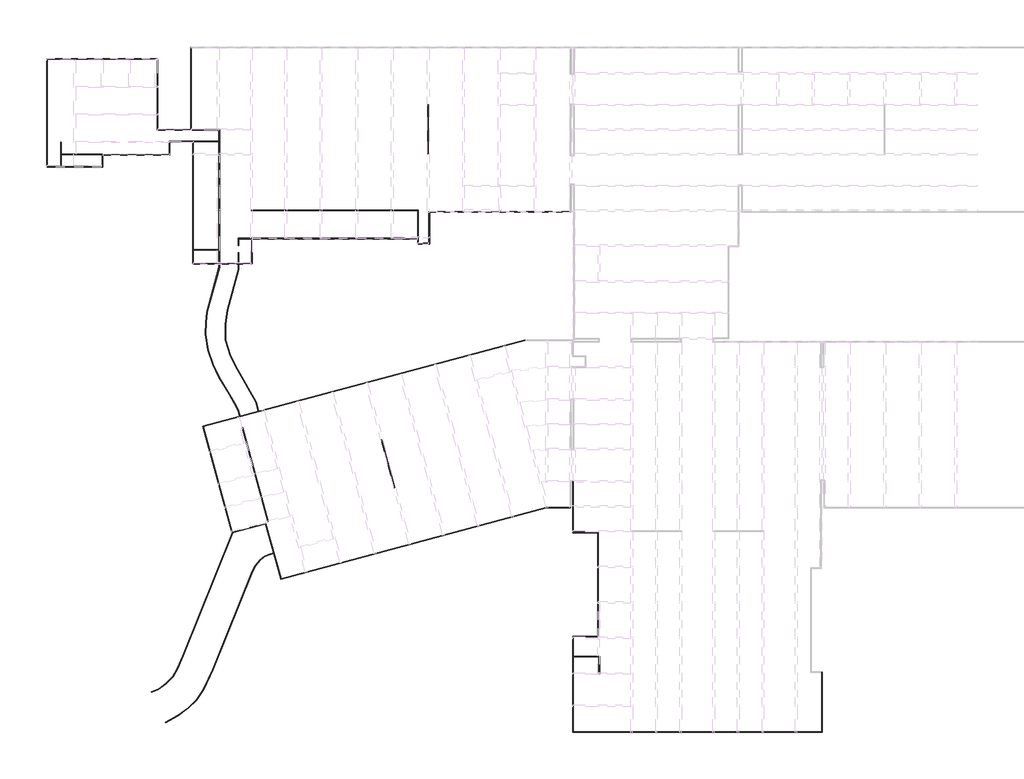
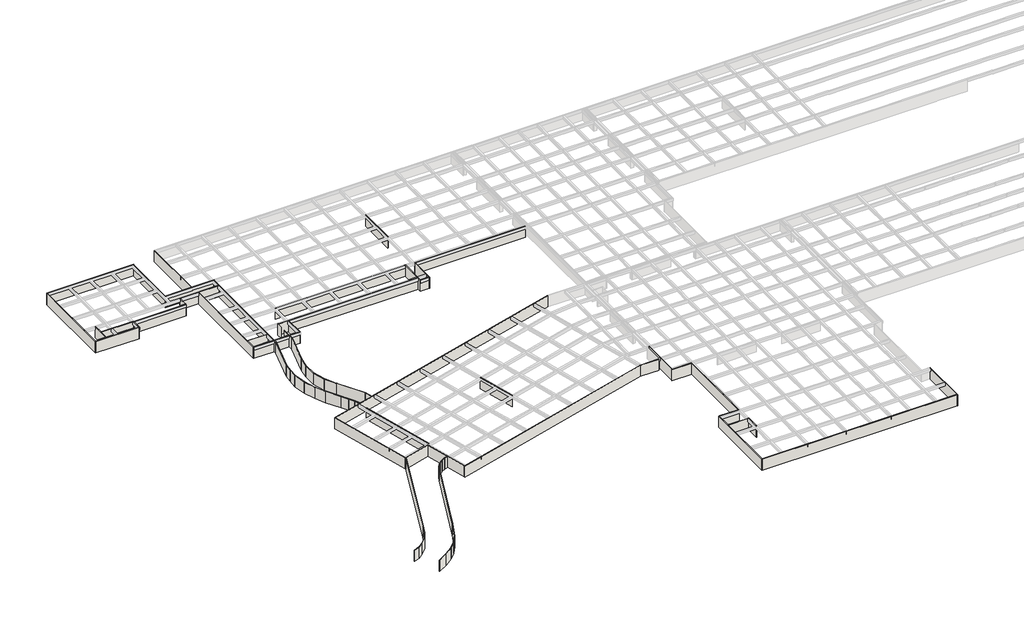
# One storey, part 1 of 14: 79 walls.
"""IFC4 building model written with IfcOpenShell, lengths in millimetres."""

from ifc_helpers import new_model, si_unit, origin, origin_with_axes, place, context, project, spatial, polyline, outline, extrude, faceted_brep, element, save

model = new_model("IFC4")

# Units and contexts
model_context = context("Model", 3, world=origin())
ifc_project = project(units=[si_unit("LENGTHUNIT", "METRE", prefix="MILLI")], contexts=[model_context])

# Site, building, storey
site = spatial("IfcSite", under=ifc_project)
building = spatial("IfcBuilding", under=site)
storey = spatial("IfcBuildingStorey", under=building, Name="户型图", Elevation=0.0)

# Walls
placement = place(None, origin())
element("IfcWall", 1, ObjectType="所有墙体", at=placement, inside=storey, context=model_context, shape_type="Brep", body=[
    faceted_brep([(-102060.8485237, -119994.1750557, 0.0), (-101940.8485237, -119994.1750557, 0.0), (-77810.8485237, -119994.1750557, 0.0), (-77690.8485237, -119994.1750557, 0.0), (-77690.8485237, -119994.1750557, 3300.0), (-77810.8485237, -119994.1750557, 3300.0), (-101940.8485237, -119994.1750557, 3300.0), (-102060.8485237, -119994.1750557, 3300.0), (-102060.8485237, -119874.1750557, 0.0), (-102060.8485237, -119874.1750557, 3300.0), (-77690.8485237, -119874.1750557, 3300.0), (-77690.8485237, -119874.1750557, 0.0)], [[[0, 1, 2, 3, 4, 5, 6, 7]], [[8, 9, 10, 11]], [[3, 2, 1, 0, 8, 11]], [[7, 6, 5, 4, 10, 9]], [[4, 3, 11, 10]], [[0, 7, 9, 8]]]),
])
element("IfcWall", 2, ObjectType="所有墙体", at=placement, inside=storey, context=model_context, shape_type="Brep", body=[
    faceted_brep([(-64072.7050956, -135348.950757, 0.0), (-70312.7050956, -135348.950757, 0.0), (-70432.7050956, -135348.950757, 0.0), (-77690.8485237, -135348.950757, 0.0), (-77810.8485237, -135348.950757, 0.0), (-77810.8485237, -135348.950757, 3300.0), (-77690.8485237, -135348.950757, 3300.0), (-70432.7050956, -135348.950757, 3300.0), (-70312.7050956, -135348.950757, 3300.0), (-64072.7050956, -135348.950757, 3300.0), (-64072.7050956, -135468.950757, 0.0), (-64072.7050956, -135468.950757, 3300.0), (-64162.6267154, -135468.950757, 3300.0), (-64282.6267154, -135468.950757, 3300.0), (-77810.8485237, -135468.950757, 3300.0), (-77810.8485237, -135468.950757, 0.0), (-64282.6267154, -135468.950757, 0.0), (-64162.6267154, -135468.950757, 0.0)], [[[0, 1, 2, 3, 4, 5, 6, 7, 8, 9]], [[10, 11, 12, 13, 14, 15, 16, 17]], [[4, 3, 2, 1, 0, 10, 17, 16, 15]], [[9, 8, 7, 6, 5, 14, 13, 12, 11]], [[0, 9, 11, 10]], [[5, 4, 15, 14]]]),
])
element("IfcWall", 3, ObjectType="所有墙体", at=placement, inside=storey, context=model_context, shape_type="SweptSolid", body=[
    extrude(outline(polyline([(-77690.8485237, -119994.1750557), (-77690.8485237, -135348.950757), (-77810.8485237, -135348.950757), (-77810.8485237, -119994.1750557), (-77690.8485237, -119994.1750557)])), origin_with_axes(), (0.0, 0.0, 1.0), 3300.0),
])
element("IfcWall", 4, ObjectType="所有墙体", at=placement, inside=storey, context=model_context, shape_type="Brep", body=[
    faceted_brep([(-64322.6267154, -137873.950757, 0.0), (-75185.8485237, -137873.950757, 0.0), (-75185.8485237, -137873.950757, 3300.0), (-64322.6267154, -137873.950757, 3300.0), (-64322.6267154, -137993.950757, 0.0), (-64322.6267154, -137993.950757, 3300.0), (-69912.7050956, -137993.950757, 3300.0), (-70032.7050956, -137993.950757, 3300.0), (-75065.8485237, -137993.950757, 3300.0), (-75185.8485237, -137993.950757, 3300.0), (-75185.8485237, -137993.950757, 0.0), (-75065.8485237, -137993.950757, 0.0), (-70032.7050956, -137993.950757, 0.0), (-69912.7050956, -137993.950757, 0.0)], [[[0, 1, 2, 3]], [[4, 5, 6, 7, 8, 9, 10, 11, 12, 13]], [[1, 0, 4, 13, 12, 11, 10]], [[3, 2, 9, 8, 7, 6, 5]], [[0, 3, 5, 4]], [[2, 1, 10, 9]]]),
])
element("IfcWall", 5, ObjectType="所有墙体", at=placement, inside=storey, context=model_context, shape_type="Brep", body=[
    faceted_brep([(-75185.8485237, -137993.950757, 0.0), (-75185.8485237, -140873.950757, 0.0), (-75185.8485237, -140993.950757, 0.0), (-75185.8485237, -140993.950757, 3300.0), (-75185.8485237, -140873.950757, 3300.0), (-75185.8485237, -137993.950757, 3300.0), (-75065.8485237, -137993.950757, 0.0), (-75065.8485237, -137993.950757, 3300.0), (-75065.8485237, -140993.950757, 3300.0), (-75065.8485237, -140993.950757, 0.0)], [[[0, 1, 2, 3, 4, 5]], [[6, 7, 8, 9]], [[2, 1, 0, 6, 9]], [[5, 4, 3, 8, 7]], [[0, 5, 7, 6]], [[3, 2, 9, 8]]]),
])
element("IfcWall", 6, ObjectType="所有墙体", at=placement, inside=storey, context=model_context, shape_type="Brep", body=[
    faceted_brep([(-75185.8485237, -140873.950757, 0.0), (-89885.8485237, -140873.950757, 0.0), (-89885.8485237, -140873.950757, 3300.0), (-75185.8485237, -140873.950757, 3300.0), (-75185.8485237, -140993.950757, 0.0), (-75185.8485237, -140993.950757, 3300.0), (-89765.8485237, -140993.950757, 3300.0), (-89885.8485237, -140993.950757, 3300.0), (-89885.8485237, -140993.950757, 0.0), (-89765.8485237, -140993.950757, 0.0)], [[[0, 1, 2, 3]], [[4, 5, 6, 7, 8, 9]], [[1, 0, 4, 9, 8]], [[3, 2, 7, 6, 5]], [[0, 3, 5, 4]], [[2, 1, 8, 7]]]),
])
element("IfcWall", 7, ObjectType="所有墙体", at=placement, inside=storey, context=model_context, shape_type="Brep", body=[
    faceted_brep([(-89885.8485237, -140993.950757, 0.0), (-89885.8485237, -143523.950757, 0.0), (-89885.8485237, -143643.950757, 0.0), (-89885.8485237, -143643.950757, 3300.0), (-89885.8485237, -143523.950757, 3300.0), (-89885.8485237, -140993.950757, 3300.0), (-89765.8485237, -140993.950757, 0.0), (-89765.8485237, -140993.950757, 3300.0), (-89765.8485237, -143643.950757, 3300.0), (-89765.8485237, -143643.950757, 0.0)], [[[0, 1, 2, 3, 4, 5]], [[6, 7, 8, 9]], [[2, 1, 0, 6, 9]], [[5, 4, 3, 8, 7]], [[0, 5, 7, 6]], [[3, 2, 9, 8]]]),
])
element("IfcWall", 8, ObjectType="所有墙体", at=placement, inside=storey, context=model_context, shape_type="Brep", body=[
    faceted_brep([(-89885.8485237, -143523.950757, 0.0), (-101940.8485237, -143523.950757, 0.0), (-102060.8485237, -143523.950757, 0.0), (-102060.8485237, -143523.950757, 3300.0), (-101940.8485237, -143523.950757, 3300.0), (-89885.8485237, -143523.950757, 3300.0), (-89885.8485237, -143643.950757, 0.0), (-89885.8485237, -143643.950757, 3300.0), (-102060.8485237, -143643.950757, 3300.0), (-102060.8485237, -143643.950757, 0.0)], [[[0, 1, 2, 3, 4, 5]], [[6, 7, 8, 9]], [[2, 1, 0, 6, 9]], [[5, 4, 3, 8, 7]], [[0, 5, 7, 6]], [[3, 2, 9, 8]]]),
])
element("IfcWall", 9, ObjectType="所有墙体", at=placement, inside=storey, context=model_context, shape_type="SweptSolid", body=[
    extrude(outline(polyline([(-101940.8485237, -119994.1750557), (-101940.8485237, -143523.950757), (-102060.8485237, -143523.950757), (-102060.8485237, -119994.1750557), (-101940.8485237, -119994.1750557)])), origin_with_axes(), (0.0, 0.0, 1.0), 3300.0),
])
element("IfcWall", 10, ObjectType="所有墙体", at=placement, inside=storey, context=model_context, shape_type="Brep", body=[
    faceted_brep([(-70312.7050956, -135348.950757, 0.0), (-70312.7050956, -117418.950757, 0.0), (-70312.7050956, -117298.950757, 0.0), (-70312.7050956, -117298.950757, 3300.0), (-70312.7050956, -117418.950757, 3300.0), (-70312.7050956, -135348.950757, 3300.0), (-70432.7050956, -135348.950757, 0.0), (-70432.7050956, -135348.950757, 3300.0), (-70432.7050956, -117298.950757, 3300.0), (-70432.7050956, -117298.950757, 0.0)], [[[0, 1, 2, 3, 4, 5]], [[6, 7, 8, 9]], [[2, 1, 0, 6, 9]], [[5, 4, 3, 8, 7]], [[0, 5, 7, 6]], [[3, 2, 9, 8]]]),
])
element("IfcWall", 11, ObjectType="所有墙体", at=placement, inside=storey, context=model_context, shape_type="Brep", body=[
    faceted_brep([(67772.2743803, -254333.1116625, 0.0), (67772.2743803, -267413.1116625, 0.0), (67772.2743803, -267533.1116625, 0.0), (67772.2743803, -267533.1116625, 3300.0), (67772.2743803, -267413.1116625, 3300.0), (67772.2743803, -254333.1116625, 3300.0), (67892.2743803, -254333.1116625, 0.0), (67892.2743803, -254333.1116625, 3300.0), (67892.2743803, -267533.1116625, 3300.0), (67892.2743803, -267533.1116625, 0.0)], [[[0, 1, 2, 3, 4, 5]], [[6, 7, 8, 9]], [[2, 1, 0, 6, 9]], [[5, 4, 3, 8, 7]], [[0, 5, 7, 6]], [[3, 2, 9, 8]]]),
])
element("IfcWall", 12, ObjectType="所有墙体", at=placement, inside=storey, context=model_context, shape_type="Brep", body=[
    faceted_brep([(67772.2743803, -267413.1116625, 0.0), (13292.2743803, -267413.1116625, 0.0), (13172.2743803, -267413.1116625, 0.0), (13172.2743803, -267413.1116625, 3300.0), (13292.2743803, -267413.1116625, 3300.0), (67772.2743803, -267413.1116625, 3300.0), (67772.2743803, -267533.1116625, 0.0), (67772.2743803, -267533.1116625, 3300.0), (13172.2743803, -267533.1116625, 3300.0), (13172.2743803, -267533.1116625, 0.0)], [[[0, 1, 2, 3, 4, 5]], [[6, 7, 8, 9]], [[2, 1, 0, 6, 9]], [[5, 4, 3, 8, 7]], [[0, 5, 7, 6]], [[3, 2, 9, 8]]]),
])
element("IfcWall", 13, ObjectType="所有墙体", at=placement, inside=storey, context=model_context, shape_type="Brep", body=[
    faceted_brep([(13292.2743803, -267413.1116625, 0.0), (13292.2743803, -250918.9547016, 0.0), (13292.2743803, -250798.9547016, 0.0), (13292.2743803, -246533.1116625, 0.0), (13292.2743803, -246413.1116625, 0.0), (13292.2743803, -246413.1116625, 3300.0), (13292.2743803, -246533.1116625, 3300.0), (13292.2743803, -250798.9547016, 3300.0), (13292.2743803, -250918.9547016, 3300.0), (13292.2743803, -267413.1116625, 3300.0), (13172.2743803, -267413.1116625, 0.0), (13172.2743803, -267413.1116625, 3300.0), (13172.2743803, -246413.1116625, 3300.0), (13172.2743803, -246413.1116625, 0.0)], [[[0, 1, 2, 3, 4, 5, 6, 7, 8, 9]], [[10, 11, 12, 13]], [[4, 3, 2, 1, 0, 10, 13]], [[9, 8, 7, 6, 5, 12, 11]], [[0, 9, 11, 10]], [[5, 4, 13, 12]]]),
])
element("IfcWall", 14, ObjectType="所有墙体", at=placement, inside=storey, context=model_context, shape_type="Brep", body=[
    faceted_brep([(13292.2743803, -246533.1116625, 0.0), (18792.2743803, -246533.1116625, 0.0), (18792.2743803, -246533.1116625, 3300.0), (13292.2743803, -246533.1116625, 3300.0), (13292.2743803, -246413.1116625, 0.0), (13292.2743803, -246413.1116625, 3300.0), (18672.2743803, -246413.1116625, 3300.0), (18792.2743803, -246413.1116625, 3300.0), (18792.2743803, -246413.1116625, 0.0), (18672.2743803, -246413.1116625, 0.0)], [[[0, 1, 2, 3]], [[4, 5, 6, 7, 8, 9]], [[1, 0, 4, 9, 8]], [[3, 2, 7, 6, 5]], [[0, 3, 5, 4]], [[2, 1, 8, 7]]]),
])
element("IfcWall", 15, ObjectType="所有墙体", at=placement, inside=storey, context=model_context, shape_type="Brep", body=[
    faceted_brep([(18792.2743803, -246413.1116625, 0.0), (18792.2743803, -223613.1116625, 0.0), (18792.2743803, -223613.1116625, 3300.0), (18792.2743803, -246413.1116625, 3300.0), (18672.2743803, -246413.1116625, 0.0), (18672.2743803, -246413.1116625, 3300.0), (18672.2743803, -223733.1116625, 3300.0), (18672.2743803, -223613.1116625, 3300.0), (18672.2743803, -223613.1116625, 0.0), (18672.2743803, -223733.1116625, 0.0)], [[[0, 1, 2, 3]], [[4, 5, 6, 7, 8, 9]], [[1, 0, 4, 9, 8]], [[3, 2, 7, 6, 5]], [[0, 3, 5, 4]], [[2, 1, 8, 7]]]),
])
element("IfcWall", 16, ObjectType="所有墙体", at=placement, inside=storey, context=model_context, shape_type="Brep", body=[
    faceted_brep([(18672.2743803, -223613.1116625, 0.0), (13292.2743803, -223613.1116625, 0.0), (13172.2743803, -223613.1116625, 0.0), (13172.2743803, -223613.1116625, 3300.0), (13292.2743803, -223613.1116625, 3300.0), (18672.2743803, -223613.1116625, 3300.0), (18672.2743803, -223733.1116625, 0.0), (18672.2743803, -223733.1116625, 3300.0), (13172.2743803, -223733.1116625, 3300.0), (13172.2743803, -223733.1116625, 0.0)], [[[0, 1, 2, 3, 4, 5]], [[6, 7, 8, 9]], [[2, 1, 0, 6, 9]], [[5, 4, 3, 8, 7]], [[0, 5, 7, 6]], [[3, 2, 9, 8]]]),
])
element("IfcWall", 17, ObjectType="所有墙体", at=placement, inside=storey, context=model_context, shape_type="Brep", body=[
    faceted_brep([(13292.2743803, -223613.1116625, 0.0), (13292.2743803, -212513.1116625, 0.0), (13292.2743803, -212513.1116625, 3300.0), (13292.2743803, -223613.1116625, 3300.0), (13172.2743803, -223613.1116625, 0.0), (13172.2743803, -223613.1116625, 3300.0), (13172.2743803, -212633.1116625, 3300.0), (13172.2743803, -212513.1116625, 3300.0), (13172.2743803, -212513.1116625, 0.0), (13172.2743803, -212633.1116625, 0.0)], [[[0, 1, 2, 3]], [[4, 5, 6, 7, 8, 9]], [[1, 0, 4, 9, 8]], [[3, 2, 7, 6, 5]], [[0, 3, 5, 4]], [[2, 1, 8, 7]]]),
])
element("IfcWall", 18, ObjectType="所有墙体", at=placement, inside=storey, context=model_context, shape_type="SweptSolid", body=[
    extrude(outline(polyline([(7424.3695711, -218205.2956278), (12672.2743803, -218205.2956278), (12672.2743803, -218325.2956278), (7440.1791895, -218325.2956278), (7424.3695711, -218205.2956278)])), origin_with_axes(), (0.0, 0.0, 1.0), 3300.0),
])
element("IfcWall", 19, ObjectType="所有墙体", at=placement, inside=storey, context=model_context, shape_type="Brep", body=[
    faceted_brep([(7424.3695711, -218205.2956278, 0.0), (-50671.4297883, -233783.5648272, 0.0), (-50787.3364124, -233814.6449502, 0.0), (-50787.3364124, -233814.6449502, 3300.0), (-50671.4297883, -233783.5648272, 3300.0), (7424.3695711, -218205.2956278, 3300.0), (7440.1791895, -218325.2956278, 0.0), (7440.1791895, -218325.2956278, 3300.0), (-50755.7106249, -233930.403877, 3300.0), (-50755.7106249, -233930.403877, 0.0)], [[[0, 1, 2, 3, 4, 5]], [[6, 7, 8, 9]], [[2, 1, 0, 6, 9]], [[5, 4, 3, 8, 7]], [[0, 5, 7, 6]], [[3, 2, 9, 8]]]),
])
element("IfcWall", 20, ObjectType="所有墙体", at=placement, inside=storey, context=model_context, shape_type="Brep", body=[
    faceted_brep([(-50671.4297883, -233783.5648272, 0.0), (-53985.8264316, -221651.9776687, 0.0), (-53985.8264316, -221651.9776687, 3300.0), (-50671.4297883, -233783.5648272, 3300.0), (-50787.3364124, -233814.6449502, 0.0), (-50787.3364124, -233814.6449502, 3300.0), (-52290.212691, -228313.7117417, 3300.0), (-52321.8387283, -228197.9519009, 3300.0), (-54070.1131044, -221798.7953563, 3300.0), (-54101.7389202, -221683.0363264, 3300.0), (-54101.7389202, -221683.0363264, 0.0), (-54070.1131044, -221798.7953563, 0.0), (-52321.8387283, -228197.9519009, 0.0), (-52290.212691, -228313.7117417, 0.0)], [[[0, 1, 2, 3]], [[4, 5, 6, 7, 8, 9, 10, 11, 12, 13]], [[1, 0, 4, 13, 12, 11, 10]], [[3, 2, 9, 8, 7, 6, 5]], [[0, 3, 5, 4]], [[2, 1, 10, 9]]]),
])
element("IfcWall", 21, ObjectType="所有墙体", at=placement, inside=storey, context=model_context, shape_type="Brep", body=[
    faceted_brep([(-54101.7389202, -221683.0363264, 0.0), (-61389.3646897, -223635.7497661, 0.0), (-61505.2771782, -223666.8084238, 0.0), (-61505.2771782, -223666.8084238, 3300.0), (-61389.3646897, -223635.7497661, 3300.0), (-54101.7389202, -221683.0363264, 3300.0), (-54070.1131044, -221798.7953563, 0.0), (-54070.1131044, -221798.7953563, 3300.0), (-61473.6513625, -223782.5674537, 3300.0), (-61473.6513625, -223782.5674537, 0.0)], [[[0, 1, 2, 3, 4, 5]], [[6, 7, 8, 9]], [[2, 1, 0, 6, 9]], [[5, 4, 3, 8, 7]], [[0, 5, 7, 6]], [[3, 2, 9, 8]]]),
])
element("IfcWall", 22, ObjectType="所有墙体", at=placement, inside=storey, context=model_context, shape_type="Brep", body=[
    faceted_brep([(-61389.3646897, -223635.7497661, 0.0), (-67709.1807348, -200503.5156291, 0.0), (-67740.8065505, -200387.7565992, 0.0), (-67740.8065505, -200387.7565992, 3300.0), (-67709.1807348, -200503.5156291, 3300.0), (-61389.3646897, -223635.7497661, 3300.0), (-61505.2771782, -223666.8084238, 0.0), (-61505.2771782, -223666.8084238, 3300.0), (-67856.719039, -200418.8152569, 3300.0), (-67856.719039, -200418.8152569, 0.0)], [[[0, 1, 2, 3, 4, 5]], [[6, 7, 8, 9]], [[2, 1, 0, 6, 9]], [[5, 4, 3, 8, 7]], [[0, 5, 7, 6]], [[3, 2, 9, 8]]]),
])
element("IfcWall", 23, ObjectType="所有墙体", at=placement, inside=storey, context=model_context, shape_type="Brep", body=[
    faceted_brep([(-67709.1807348, -200503.5156291, 0.0), (2737.534582, -181627.3751505, 0.0), (2737.534582, -181627.3751505, 3300.0), (-67709.1807348, -200503.5156291, 3300.0), (-67740.8065505, -200387.7565992, 0.0), (-67740.8065505, -200387.7565992, 3300.0), (-59754.9827385, -198247.9615579, 3300.0), (-59639.0716393, -198216.9032725, 3300.0), (-55640.8160452, -197145.5739149, 3300.0), (-55524.904946, -197114.5156295, 3300.0), (2721.7362823, -181507.3751505, 3300.0), (2721.7362823, -181507.3751505, 0.0), (-55524.904946, -197114.5156295, 0.0), (-55640.8160452, -197145.5739149, 0.0), (-59639.0716393, -198216.9032725, 0.0), (-59754.9827385, -198247.9615579, 0.0)], [[[0, 1, 2, 3]], [[4, 5, 6, 7, 8, 9, 10, 11, 12, 13, 14, 15]], [[1, 0, 4, 15, 14, 13, 12, 11]], [[3, 2, 10, 9, 8, 7, 6, 5]], [[0, 3, 5, 4]], [[2, 1, 11, 10]]]),
])
element("IfcWall", 24, ObjectType="所有墙体", at=placement, inside=storey, context=model_context, shape_type="Brep", body=[
    faceted_brep([(12717.2949044, -153307.3751505, 0.0), (-18282.7050956, -153307.3751505, 0.0), (-18282.7050956, -153307.3751505, 3300.0), (12717.2949044, -153307.3751505, 3300.0), (12717.2949044, -153427.3751505, 0.0), (12717.2949044, -153427.3751505, 3300.0), (-18162.7050956, -153427.3751505, 3300.0), (-18282.7050956, -153427.3751505, 3300.0), (-18282.7050956, -153427.3751505, 0.0), (-18162.7050956, -153427.3751505, 0.0)], [[[0, 1, 2, 3]], [[4, 5, 6, 7, 8, 9]], [[1, 0, 4, 9, 8]], [[3, 2, 7, 6, 5]], [[0, 3, 5, 4]], [[2, 1, 8, 7]]]),
])
element("IfcWall", 25, ObjectType="所有墙体", at=placement, inside=storey, context=model_context, shape_type="Brep", body=[
    faceted_brep([(-18282.7050956, -153427.3751505, 0.0), (-18282.7050956, -160307.3751505, 0.0), (-18282.7050956, -160427.3751505, 0.0), (-18282.7050956, -160427.3751505, 3300.0), (-18282.7050956, -160307.3751505, 3300.0), (-18282.7050956, -153427.3751505, 3300.0), (-18162.7050956, -153427.3751505, 0.0), (-18162.7050956, -153427.3751505, 3300.0), (-18162.7050956, -160427.3751505, 3300.0), (-18162.7050956, -160427.3751505, 0.0)], [[[0, 1, 2, 3, 4, 5]], [[6, 7, 8, 9]], [[2, 1, 0, 6, 9]], [[5, 4, 3, 8, 7]], [[0, 5, 7, 6]], [[3, 2, 9, 8]]]),
])
element("IfcWall", 26, ObjectType="所有墙体", at=placement, inside=storey, context=model_context, shape_type="Brep", body=[
    faceted_brep([(-18282.7050956, -160307.3751505, 0.0), (-20662.7050956, -160307.3751505, 0.0), (-20782.7050956, -160307.3751505, 0.0), (-20782.7050956, -160307.3751505, 3300.0), (-20662.7050956, -160307.3751505, 3300.0), (-18282.7050956, -160307.3751505, 3300.0), (-18282.7050956, -160427.3751505, 0.0), (-18282.7050956, -160427.3751505, 3300.0), (-20782.7050956, -160427.3751505, 3300.0), (-20782.7050956, -160427.3751505, 0.0)], [[[0, 1, 2, 3, 4, 5]], [[6, 7, 8, 9]], [[2, 1, 0, 6, 9]], [[5, 4, 3, 8, 7]], [[0, 5, 7, 6]], [[3, 2, 9, 8]]]),
])
element("IfcWall", 27, ObjectType="所有墙体", at=placement, inside=storey, context=model_context, shape_type="Brep", body=[
    faceted_brep([(-20662.7050956, -160307.3751505, 0.0), (-20662.7050956, -153048.950757, 0.0), (-20662.7050956, -153048.950757, 3300.0), (-20662.7050956, -160307.3751505, 3300.0), (-20782.7050956, -160307.3751505, 0.0), (-20782.7050956, -160307.3751505, 3300.0), (-20782.7050956, -159327.3751505, 3300.0), (-20782.7050956, -159207.3751505, 3300.0), (-20782.7050956, -153168.950757, 3300.0), (-20782.7050956, -153048.950757, 3300.0), (-20782.7050956, -153048.950757, 0.0), (-20782.7050956, -153168.950757, 0.0), (-20782.7050956, -159207.3751505, 0.0), (-20782.7050956, -159327.3751505, 0.0)], [[[0, 1, 2, 3]], [[4, 5, 6, 7, 8, 9, 10, 11, 12, 13]], [[1, 0, 4, 13, 12, 11, 10]], [[3, 2, 9, 8, 7, 6, 5]], [[0, 3, 5, 4]], [[2, 1, 10, 9]]]),
])
element("IfcWall", 28, ObjectType="所有墙体", at=placement, inside=storey, context=model_context, shape_type="Brep", body=[
    faceted_brep([(-20782.7050956, -159207.3751505, 0.0), (-59913.7017341, -159207.3751505, 0.0), (-59913.7017341, -159207.3751505, 3300.0), (-20782.7050956, -159207.3751505, 3300.0), (-20782.7050956, -159327.3751505, 0.0), (-20782.7050956, -159327.3751505, 3300.0), (-56962.7050956, -159327.3751505, 3300.0), (-57082.7050956, -159327.3751505, 3300.0), (-59913.7017341, -159327.3751505, 3300.0), (-59913.7017341, -159327.3751505, 0.0), (-57082.7050956, -159327.3751505, 0.0), (-56962.7050956, -159327.3751505, 0.0)], [[[0, 1, 2, 3]], [[4, 5, 6, 7, 8, 9, 10, 11]], [[1, 0, 4, 11, 10, 9]], [[3, 2, 8, 7, 6, 5]], [[0, 3, 5, 4]], [[2, 1, 9, 8]]]),
])
element("IfcWall", 29, ObjectType="所有墙体", at=placement, inside=storey, context=model_context, shape_type="Brep", body=[
    faceted_brep([(-57082.7050956, -159327.3751505, 0.0), (-57082.7050956, -164698.4277999, 0.0), (-57082.7050956, -164818.4277999, 0.0), (-57082.7050956, -164818.4277999, 3300.0), (-57082.7050956, -164698.4277999, 3300.0), (-57082.7050956, -159327.3751505, 3300.0), (-56962.7050956, -159327.3751505, 0.0), (-56962.7050956, -159327.3751505, 3300.0), (-56962.7050956, -164818.4277999, 3300.0), (-56962.7050956, -164818.4277999, 0.0)], [[[0, 1, 2, 3, 4, 5]], [[6, 7, 8, 9]], [[2, 1, 0, 6, 9]], [[5, 4, 3, 8, 7]], [[0, 5, 7, 6]], [[3, 2, 9, 8]]]),
])
element("IfcWall", 30, ObjectType="所有墙体", at=placement, inside=storey, context=model_context, shape_type="Brep", body=[
    faceted_brep([(-57082.7050956, -164698.4277999, 0.0), (-59950.6326698, -164698.4277999, 0.0), (-60070.6326698, -164698.4277999, 0.0), (-64162.6267154, -164698.4277999, 0.0), (-64282.6267154, -164698.4277999, 0.0), (-69912.7050956, -164698.4277999, 0.0), (-70032.7050956, -164698.4277999, 0.0), (-70032.7050956, -164698.4277999, 3300.0), (-69912.7050956, -164698.4277999, 3300.0), (-64282.6267154, -164698.4277999, 3300.0), (-64162.6267154, -164698.4277999, 3300.0), (-60070.6326698, -164698.4277999, 3300.0), (-59950.6326698, -164698.4277999, 3300.0), (-57082.7050956, -164698.4277999, 3300.0), (-57082.7050956, -164818.4277999, 0.0), (-57082.7050956, -164818.4277999, 3300.0), (-59950.6326698, -164818.4277999, 3300.0), (-60070.6326698, -164818.4277999, 3300.0), (-64162.6267154, -164818.4277999, 3300.0), (-64282.6267154, -164818.4277999, 3300.0), (-70032.7050956, -164818.4277999, 3300.0), (-70032.7050956, -164818.4277999, 0.0), (-64282.6267154, -164818.4277999, 0.0), (-64162.6267154, -164818.4277999, 0.0), (-60070.6326698, -164818.4277999, 0.0), (-59950.6326698, -164818.4277999, 0.0)], [[[0, 1, 2, 3, 4, 5, 6, 7, 8, 9, 10, 11, 12, 13]], [[14, 15, 16, 17, 18, 19, 20, 21, 22, 23, 24, 25]], [[6, 5, 4, 3, 2, 1, 0, 14, 25, 24, 23, 22, 21]], [[13, 12, 11, 10, 9, 8, 7, 20, 19, 18, 17, 16, 15]], [[0, 13, 15, 14]], [[7, 6, 21, 20]]]),
])
element("IfcWall", 31, ObjectType="所有墙体", at=placement, inside=storey, context=model_context, shape_type="Brep", body=[
    faceted_brep([(-69912.7050956, -164698.4277999, 0.0), (-69912.7050956, -161762.6341765, 0.0), (-69912.7050956, -161642.6341765, 0.0), (-69912.7050956, -137993.950757, 0.0), (-69912.7050956, -137993.950757, 3300.0), (-69912.7050956, -161642.6341765, 3300.0), (-69912.7050956, -161762.6341765, 3300.0), (-69912.7050956, -164698.4277999, 3300.0), (-70032.7050956, -164698.4277999, 0.0), (-70032.7050956, -164698.4277999, 3300.0), (-70032.7050956, -137993.950757, 3300.0), (-70032.7050956, -137993.950757, 0.0)], [[[0, 1, 2, 3, 4, 5, 6, 7]], [[8, 9, 10, 11]], [[3, 2, 1, 0, 8, 11]], [[7, 6, 5, 4, 10, 9]], [[0, 7, 9, 8]], [[4, 3, 11, 10]]]),
])
element("IfcWall", 32, ObjectType="所有墙体", at=placement, inside=storey, context=model_context, shape_type="SweptSolid", body=[
    extrude(outline(polyline([(-25928.9541564, -213876.8076269), (-28736.3690064, -203399.4100936), (-28620.4579201, -203368.3517603), (-25813.0430701, -213845.7492935), (-25928.9541564, -213876.8076269)])), origin_with_axes(), (0.0, 0.0, 1.0), 3300.0),
])
element("IfcWall", 33, ObjectType="所有墙体", at=placement, inside=storey, context=model_context, shape_type="SweptSolid", body=[
    extrude(outline(polyline([(-18534.1452268, -140660.1299915), (-18534.1452268, -129960.1299915), (-18414.1452268, -129960.1299915), (-18414.1452268, -140660.1299915), (-18534.1452268, -140660.1299915)])), origin_with_axes(), (0.0, 0.0, 1.0), 3300.0),
])
element("IfcWall", 34, ObjectType="所有墙体", at=placement, inside=storey, context=model_context, shape_type="SweptSolid", body=[
    extrude(outline(polyline([(-57172.7050956, -153048.950757), (-20782.7050956, -153048.950757), (-20782.7050956, -153168.950757), (-57172.7050956, -153168.950757), (-57172.7050956, -153048.950757)])), origin_with_axes(), (0.0, 0.0, 1.0), 3300.0),
])
element("IfcWall", 35, ObjectType="所有墙体", at=placement, inside=storey, context=model_context, shape_type="Brep", body=[
    faceted_brep([(-64282.6267154, -135468.950757, 0.0), (-64282.6267154, -161642.6341765, 0.0), (-64282.6267154, -161762.6341765, 0.0), (-64282.6267154, -164698.4277999, 0.0), (-64282.6267154, -164698.4277999, 3300.0), (-64282.6267154, -161762.6341765, 3300.0), (-64282.6267154, -161642.6341765, 3300.0), (-64282.6267154, -135468.950757, 3300.0), (-64162.6267154, -135468.950757, 0.0), (-64162.6267154, -135468.950757, 3300.0), (-64162.6267154, -164698.4277999, 3300.0), (-64162.6267154, -164698.4277999, 0.0)], [[[0, 1, 2, 3, 4, 5, 6, 7]], [[8, 9, 10, 11]], [[3, 2, 1, 0, 8, 11]], [[7, 6, 5, 4, 10, 9]], [[0, 7, 9, 8]], [[4, 3, 11, 10]]]),
])
element("IfcWall", 36, ObjectType="所有墙体", at=placement, inside=storey, context=model_context, shape_type="SweptSolid", body=[
    extrude(outline(polyline([(-69912.7050956, -161642.6341765), (-64282.6267154, -161642.6341765), (-64282.6267154, -161762.6341765), (-69912.7050956, -161762.6341765), (-69912.7050956, -161642.6341765)])), origin_with_axes(), (0.0, 0.0, 1.0), 3300.0),
])
element("IfcWall", 37, ObjectType="所有墙体", at=placement, inside=storey, context=model_context, shape_type="SweptSolid", body=[
    extrude(outline(polyline([(-64282.6267154, -165550.52865), (-64282.6267154, -164818.4277999), (-64162.6267154, -164818.4277999), (-64162.6267154, -165566.3269497), (-64282.6267154, -165550.52865)])), origin_with_axes(), (0.0, 0.0, 1.0), 3300.0),
])
element("IfcWall", 38, ObjectType="所有墙体", at=placement, inside=storey, context=model_context, shape_type="SweptSolid", body=[
    extrude(outline(polyline([(-66921.7586951, -175399.903286), (-64282.6267154, -165550.52865), (-64162.6267154, -165566.3269497), (-66803.4032558, -175421.83917), (-66921.7586951, -175399.903286)])), origin_with_axes(), (0.0, 0.0, 1.0), 3300.0),
])
element("IfcWall", 39, ObjectType="所有墙体", at=placement, inside=storey, context=model_context, shape_type="SweptSolid", body=[
    extrude(outline(polyline([(-67162.8319851, -177693.5624279), (-66921.7586951, -175399.903286), (-66803.4032558, -175421.83917), (-67043.1608968, -177702.9807468), (-67162.8319851, -177693.5624279)])), origin_with_axes(), (0.0, 0.0, 1.0), 3300.0),
])
element("IfcWall", 40, ObjectType="所有墙体", at=placement, inside=storey, context=model_context, shape_type="SweptSolid", body=[
    extrude(outline(polyline([(-67291.9097037, -180156.5120195), (-67162.8319851, -177693.5624279), (-67043.1608968, -177702.9807468), (-67171.4140719, -180150.197111), (-67291.9097037, -180156.5120195)])), origin_with_axes(), (0.0, 0.0, 1.0), 3300.0),
])
element("IfcWall", 41, ObjectType="所有墙体", at=placement, inside=storey, context=model_context, shape_type="SweptSolid", body=[
    extrude(outline(polyline([(-66726.9816527, -183723.3273571), (-67291.9097037, -180156.5120195), (-67171.4140719, -180150.197111), (-66610.0139746, -183694.7378257), (-66726.9816527, -183723.3273571)])), origin_with_axes(), (0.0, 0.0, 1.0), 3300.0),
])
element("IfcWall", 42, ObjectType="所有墙体", at=placement, inside=storey, context=model_context, shape_type="SweptSolid", body=[
    extrude(outline(polyline([(-65678.7698235, -186861.5323686), (-66726.9816527, -183723.3273571), (-66610.0139746, -183694.7378257), (-65567.2747284, -186816.5586607), (-65678.7698235, -186861.5323686)])), origin_with_axes(), (0.0, 0.0, 1.0), 3300.0),
])
element("IfcWall", 43, ObjectType="所有墙体", at=placement, inside=storey, context=model_context, shape_type="SweptSolid", body=[
    extrude(outline(polyline([(-64343.0654647, -189666.2881503), (-65678.7698235, -186861.5323686), (-65567.2747284, -186816.5586607), (-64237.2178441, -189609.4556902), (-64343.0654647, -189666.2881503)])), origin_with_axes(), (0.0, 0.0, 1.0), 3300.0),
])
element("IfcWall", 44, ObjectType="所有墙体", at=placement, inside=storey, context=model_context, shape_type="SweptSolid", body=[
    extrude(outline(polyline([(-62055.07232, -193474.1481968), (-64343.0654647, -189666.2881503), (-64237.2178441, -189609.4556902), (-61951.6728836, -193413.241274), (-62055.07232, -193474.1481968)])), origin_with_axes(), (0.0, 0.0, 1.0), 3300.0),
])
element("IfcWall", 45, ObjectType="所有墙体", at=placement, inside=storey, context=model_context, shape_type="SweptSolid", body=[
    extrude(outline(polyline([(-60955.4254517, -195378.7924431), (-62055.07232, -193474.1481967), (-61951.6728836, -193413.241274), (-60851.3197519, -195319.1088044), (-60955.4254517, -195378.7924431)])), origin_with_axes(), (0.0, 0.0, 1.0), 3300.0),
])
element("IfcWall", 46, ObjectType="所有墙体", at=placement, inside=storey, context=model_context, shape_type="SweptSolid", body=[
    extrude(outline(polyline([(-60139.9172399, -196811.3664409), (-60955.4254517, -195378.7924431), (-60851.3197519, -195319.1088044), (-60027.9988942, -196765.406997), (-60139.9172399, -196811.3664409)])), origin_with_axes(), (0.0, 0.0, 1.0), 3300.0),
])
element("IfcWall", 47, ObjectType="所有墙体", at=placement, inside=storey, context=model_context, shape_type="SweptSolid", body=[
    extrude(outline(polyline([(-59754.9827385, -198247.9615579), (-60139.9172399, -196811.3664409), (-60027.9988942, -196765.406997), (-59639.0716393, -198216.9032725), (-59754.9827385, -198247.9615579)])), origin_with_axes(), (0.0, 0.0, 1.0), 3300.0),
])
element("IfcWall", 48, ObjectType="所有墙体", at=placement, inside=storey, context=model_context, shape_type="SweptSolid", body=[
    extrude(outline(polyline([(-56080.8229941, -195039.8045814), (-55524.904946, -197114.5156295), (-55640.8160452, -197145.5739149), (-56192.6451801, -195086.1228739), (-56080.8229941, -195039.8045814)])), origin_with_axes(), (0.0, 0.0, 1.0), 3300.0),
])
element("IfcWall", 49, ObjectType="所有墙体", at=placement, inside=storey, context=model_context, shape_type="SweptSolid", body=[
    extrude(outline(polyline([(-60184.3356946, -187932.3120946), (-56080.8229941, -195039.8045814), (-56192.6451801, -195086.1228739), (-60289.1324796, -187990.7987386), (-60184.3356946, -187932.3120946)])), origin_with_axes(), (0.0, 0.0, 1.0), 3300.0),
])
element("IfcWall", 50, ObjectType="所有墙体", at=placement, inside=storey, context=model_context, shape_type="SweptSolid", body=[
    extrude(outline(polyline([(-61755.993167, -185017.256202), (-60184.3356946, -187932.3120946), (-60289.1324796, -187990.7987386), (-61867.4848403, -185063.3253989), (-61755.993167, -185017.256202)])), origin_with_axes(), (0.0, 0.0, 1.0), 3300.0),
])
element("IfcWall", 51, ObjectType="所有墙体", at=placement, inside=storey, context=model_context, shape_type="SweptSolid", body=[
    extrude(outline(polyline([(-62816.7147264, -181452.3559054), (-61755.993167, -185017.256202), (-61867.4848403, -185063.3253989), (-62936.7147264, -181469.830099), (-62816.7147264, -181452.3559054)])), origin_with_axes(), (0.0, 0.0, 1.0), 3300.0),
])
element("IfcWall", 52, ObjectType="所有墙体", at=placement, inside=storey, context=model_context, shape_type="SweptSolid", body=[
    extrude(outline(polyline([(-62816.7147264, -177965.8151046), (-62816.7147264, -181452.3559054), (-62936.7147264, -181469.830099), (-62936.7147264, -177956.3708998), (-62816.7147264, -177965.8151046)])), origin_with_axes(), (0.0, 0.0, 1.0), 3300.0),
])
element("IfcWall", 53, ObjectType="所有墙体", at=placement, inside=storey, context=model_context, shape_type="SweptSolid", body=[
    extrude(outline(polyline([(-62332.9984873, -174911.7509674), (-62816.7147264, -177965.8151046), (-62936.7147264, -177956.3708998), (-62450.5372822, -174886.7673253), (-62332.9984873, -174911.7509674)])), origin_with_axes(), (0.0, 0.0, 1.0), 3300.0),
])
element("IfcWall", 54, ObjectType="所有墙体", at=placement, inside=storey, context=model_context, shape_type="SweptSolid", body=[
    extrude(outline(polyline([(-59950.6326698, -166020.6406944), (-62332.9984873, -174911.7509674), (-62450.5372822, -174886.7673253), (-60070.6326698, -166004.8423946), (-59950.6326698, -166020.6406944)])), origin_with_axes(), (0.0, 0.0, 1.0), 3300.0),
])
element("IfcWall", 55, ObjectType="所有墙体", at=placement, inside=storey, context=model_context, shape_type="SweptSolid", body=[
    extrude(outline(polyline([(-59950.6326698, -164818.4277999), (-59950.6326698, -166020.6406944), (-60070.6326698, -166004.8423946), (-60070.6326698, -164818.4277999), (-59950.6326698, -164818.4277999)])), origin_with_axes(), (0.0, 0.0, 1.0), 3300.0),
])
element("IfcWall", 56, ObjectType="所有墙体", at=placement, inside=storey, context=model_context, shape_type="SweptSolid", body=[
    extrude(outline(polyline([(-59950.6326698, -162357.0185835), (-59950.6326698, -164698.4277999), (-60070.6326698, -164698.4277999), (-60070.6326698, -162357.0185835), (-59950.6326698, -162357.0185835)])), origin_with_axes(), (0.0, 0.0, 1.0), 3300.0),
])
element("IfcWall", 57, ObjectType="所有墙体", at=placement, inside=storey, context=model_context, shape_type="Brep", body=[
    faceted_brep([(-59913.7017341, -160829.181821, 0.0), (-59913.7017341, -159327.3751505, 0.0), (-59913.7017341, -159207.3751505, 0.0), (-59913.7017341, -159189.181821, 0.0), (-59913.7017341, -159189.181821, 3300.0), (-59913.7017341, -159207.3751505, 3300.0), (-59913.7017341, -159327.3751505, 3300.0), (-59913.7017341, -160829.181821, 3300.0), (-60033.7017341, -160829.181821, 0.0), (-60033.7017341, -160829.181821, 3300.0), (-60033.7017341, -159189.181821, 3300.0), (-60033.7017341, -159189.181821, 0.0)], [[[0, 1, 2, 3, 4, 5, 6, 7]], [[8, 9, 10, 11]], [[3, 2, 1, 0, 8, 11]], [[4, 3, 11, 10]], [[7, 6, 5, 4, 10, 9]], [[0, 7, 9, 8]]]),
])
element("IfcWall", 58, ObjectType="所有墙体", at=placement, inside=storey, context=model_context, shape_type="SweptSolid", body=[
    extrude(outline(polyline([(-59074.9933121, -200705.199268), (-53479.354271, -221257.0562089), (-53595.1393805, -221288.5809359), (-59190.7784216, -200736.723995), (-59074.9933121, -200705.199268)])), origin_with_axes(), (0.0, 0.0, 1.0), 3300.0),
])
element("IfcWall", 59, ObjectType="所有墙体", at=placement, inside=storey, context=model_context, shape_type="SweptSolid", body=[
    extrude(outline(polyline([(-53332.1758898, -228467.2995997), (-52321.8387283, -228197.9519009), (-52290.212691, -228313.7117417), (-53289.6794099, -228580.1614685), (-53332.1758898, -228467.2995997)])), origin_with_axes(), (0.0, 0.0, 1.0), 3300.0),
])
element("IfcWall", 60, ObjectType="所有墙体", at=placement, inside=storey, context=model_context, shape_type="SweptSolid", body=[
    extrude(outline(polyline([(-54384.4165476, -228988.2371362), (-53332.1758898, -228467.2995997), (-53289.6794099, -228580.1614685), (-54323.0312208, -229091.7476183), (-54384.4165476, -228988.2371362)])), origin_with_axes(), (0.0, 0.0, 1.0), 3300.0),
])
element("IfcWall", 61, ObjectType="所有墙体", at=placement, inside=storey, context=model_context, shape_type="SweptSolid", body=[
    extrude(outline(polyline([(-55378.8225506, -229684.5277155), (-54384.4165476, -228988.2371362), (-54323.0312208, -229091.7476183), (-55294.5901241, -229772.0404862), (-55378.8225506, -229684.5277155)])), origin_with_axes(), (0.0, 0.0, 1.0), 3300.0),
])
element("IfcWall", 62, ObjectType="所有墙体", at=placement, inside=storey, context=model_context, shape_type="SweptSolid", body=[
    extrude(outline(polyline([(-56324.7466149, -230931.2588895), (-55378.8225506, -229684.5277155), (-55294.5901241, -229772.0404862), (-56222.6824012, -230995.2693031), (-56324.7466149, -230931.2588895)])), origin_with_axes(), (0.0, 0.0, 1.0), 3300.0),
])
element("IfcWall", 63, ObjectType="所有墙体", at=placement, inside=storey, context=model_context, shape_type="SweptSolid", body=[
    extrude(outline(polyline([(-56945.801356, -232150.1474488), (-56324.7466149, -230931.2588895), (-56222.6824012, -230995.2693031), (-56836.4818194, -232199.9184896), (-56945.801356, -232150.1474488)])), origin_with_axes(), (0.0, 0.0, 1.0), 3300.0),
])
element("IfcWall", 64, ObjectType="所有墙体", at=placement, inside=storey, context=model_context, shape_type="SweptSolid", body=[
    extrude(outline(polyline([(-65621.1781702, -253668.1977776), (-56945.801356, -232150.1474488), (-56836.4818194, -232199.9184896), (-65511.0744984, -253716.0238814), (-65621.1781702, -253668.1977776)])), origin_with_axes(), (0.0, 0.0, 1.0), 3300.0),
])
element("IfcWall", 65, ObjectType="所有墙体", at=placement, inside=storey, context=model_context, shape_type="SweptSolid", body=[
    extrude(outline(polyline([(-67689.1158257, -258102.9043908), (-65621.1781702, -253668.1977776), (-65511.0744984, -253716.0238814), (-67584.7958081, -258163.1335811), (-67689.1158257, -258102.9043908)])), origin_with_axes(), (0.0, 0.0, 1.0), 3300.0),
])
element("IfcWall", 66, ObjectType="所有墙体", at=placement, inside=storey, context=model_context, shape_type="SweptSolid", body=[
    extrude(outline(polyline([(-69289.1080751, -260387.9301327), (-67689.1158257, -258102.9043908), (-67584.7958081, -258163.1335811), (-69196.8316021, -260465.3592872), (-69289.1080751, -260387.9301327)])), origin_with_axes(), (0.0, 0.0, 1.0), 3300.0),
])
element("IfcWall", 67, ObjectType="所有墙体", at=placement, inside=storey, context=model_context, shape_type="SweptSolid", body=[
    extrude(outline(polyline([(-70979.485777, -262078.3078346), (-69289.1080751, -260387.9301327), (-69196.8316021, -260465.3592872), (-70900.56645, -262169.0941351), (-70979.485777, -262078.3078346)])), origin_with_axes(), (0.0, 0.0, 1.0), 3300.0),
])
element("IfcWall", 68, ObjectType="所有墙体", at=placement, inside=storey, context=model_context, shape_type="SweptSolid", body=[
    extrude(outline(polyline([(-73288.4067553, -263818.2045892), (-70979.485777, -262078.3078346), (-70900.56645, -262169.0941351), (-73223.7314299, -263919.7245147), (-73288.4067553, -263818.2045892)])), origin_with_axes(), (0.0, 0.0, 1.0), 3300.0),
])
element("IfcWall", 69, ObjectType="所有墙体", at=placement, inside=storey, context=model_context, shape_type="SweptSolid", body=[
    extrude(outline(polyline([(-76006.9655566, -265263.6879444), (-73288.4067553, -263818.2045892), (-73223.7314299, -263919.7245147), (-75950.6289691, -265369.6416555), (-76006.9655566, -265263.6879444)])), origin_with_axes(), (0.0, 0.0, 1.0), 3300.0),
])
element("IfcWall", 70, ObjectType="所有墙体", at=placement, inside=storey, context=model_context, shape_type="SweptSolid", body=[
    extrude(outline(polyline([(-77459.9211506, -258084.6752988), (-79054.880246, -258696.9227329), (-79097.8843999, -258584.8930817), (-77518.6700452, -257978.6894873), (-77459.9211506, -258084.6752988)])), origin_with_axes(), (0.0, 0.0, 1.0), 3300.0),
])
element("IfcWall", 71, ObjectType="所有墙体", at=placement, inside=storey, context=model_context, shape_type="SweptSolid", body=[
    extrude(outline(polyline([(-75852.5649143, -256873.445497), (-77459.9211506, -258084.6752988), (-77518.6700452, -257978.6894873), (-75931.4842413, -256782.6591965), (-75852.5649143, -256873.445497)])), origin_with_axes(), (0.0, 0.0, 1.0), 3300.0),
])
element("IfcWall", 72, ObjectType="所有墙体", at=placement, inside=storey, context=model_context, shape_type="SweptSolid", body=[
    extrude(outline(polyline([(-74288.3777099, -255309.2582926), (-75852.5649143, -256873.445497), (-75931.4842413, -256782.6591965), (-74384.4016085, -255235.5765637), (-74288.3777099, -255309.2582926)])), origin_with_axes(), (0.0, 0.0, 1.0), 3300.0),
])
element("IfcWall", 73, ObjectType="所有墙体", at=placement, inside=storey, context=model_context, shape_type="SweptSolid", body=[
    extrude(outline(polyline([(-73282.3191985, -253566.7138355), (-74288.3777099, -255309.2582926), (-74384.4016085, -255235.5765637), (-73390.4601199, -253514.0194057), (-73282.3191985, -253566.7138355)])), origin_with_axes(), (0.0, 0.0, 1.0), 3300.0),
])
element("IfcWall", 74, ObjectType="所有墙体", at=placement, inside=storey, context=model_context, shape_type="SweptSolid", body=[
    extrude(outline(polyline([(-72158.9767751, -250780.4211682), (-73282.3191985, -253566.7138355), (-73390.4601199, -253514.0194057), (-72270.2720054, -250735.5505574), (-72158.9767751, -250780.4211682)])), origin_with_axes(), (0.0, 0.0, 1.0), 3300.0),
])
element("IfcWall", 75, ObjectType="所有墙体", at=placement, inside=storey, context=model_context, shape_type="SweptSolid", body=[
    extrude(outline(polyline([(-61256.5842644, -223799.9637432), (-72158.9944906, -250780.4650591), (-72270.2542899, -250735.5066664), (-61367.8440637, -223755.0053505), (-61256.5842644, -223799.9637432)])), origin_with_axes(), (0.0, 0.0, 1.0), 3300.0),
])
element("IfcWall", 76, ObjectType="所有墙体", at=placement, inside=storey, context=model_context, shape_type="Brep", body=[
    faceted_brep([(-98935.8485237, -138112.0857972, 0.0), (-98935.8485237, -143212.0857972, 0.0), (-98935.8485237, -143212.0857972, 3300.0), (-98935.8485237, -138112.0857972, 3300.0), (-98815.8485237, -138112.0857972, 0.0), (-98815.8485237, -138112.0857972, 3300.0), (-98815.8485237, -140703.950757, 3300.0), (-98815.8485237, -140823.950757, 3300.0), (-98815.8485237, -143212.0857972, 3300.0), (-98815.8485237, -143212.0857972, 0.0), (-98815.8485237, -140823.950757, 0.0), (-98815.8485237, -140703.950757, 0.0)], [[[0, 1, 2, 3]], [[4, 5, 6, 7, 8, 9, 10, 11]], [[1, 0, 4, 11, 10, 9]], [[2, 1, 9, 8]], [[3, 2, 8, 7, 6, 5]], [[0, 3, 5, 4]]]),
])
element("IfcWall", 77, ObjectType="所有墙体", at=placement, inside=storey, context=model_context, shape_type="SweptSolid", body=[
    extrude(outline(polyline([(-89825.8485237, -140823.950757), (-98815.8485237, -140823.950757), (-98815.8485237, -140703.950757), (-89825.8485237, -140703.950757), (-89825.8485237, -140823.950757)])), origin_with_axes(), (0.0, 0.0, 1.0), 3300.0),
])
element("IfcWall", 78, ObjectType="所有墙体", at=placement, inside=storey, context=model_context, shape_type="Brep", body=[
    faceted_brep([(13292.2743803, -250918.9547016, 0.0), (18967.2949044, -250918.9547016, 0.0), (19087.2949044, -250918.9547016, 0.0), (19087.2949044, -250918.9547016, 3300.0), (18967.2949044, -250918.9547016, 3300.0), (13292.2743803, -250918.9547016, 3300.0), (13292.2743803, -250798.9547016, 0.0), (13292.2743803, -250798.9547016, 3300.0), (19087.2949044, -250798.9547016, 3300.0), (19087.2949044, -250798.9547016, 0.0)], [[[0, 1, 2, 3, 4, 5]], [[6, 7, 8, 9]], [[2, 1, 0, 6, 9]], [[5, 4, 3, 8, 7]], [[0, 5, 7, 6]], [[3, 2, 9, 8]]]),
])
element("IfcWall", 79, ObjectType="所有墙体", at=placement, inside=storey, context=model_context, shape_type="SweptSolid", body=[
    extrude(outline(polyline([(18967.2949044, -254662.9547016), (18967.2949044, -250918.9547016), (19087.2949044, -250918.9547016), (19087.2949044, -254662.9547016), (18967.2949044, -254662.9547016)])), origin_with_axes(), (0.0, 0.0, 1.0), 3300.0),
])

save(model, "model.ifc")

# Revit data of these elements
# Project information
#   项目发布日期 = "出图日期"
#   项目状态 = "项目状态"
#   客户姓名 = "所有者"
#   项目地址 = "## 街道\n省市自治区邮政编码"
#   项目名称 = "项目名称"
#   项目编号 = "项目编号"
# Type "所有墙体"
#   Layers, outside or top first: 120 mm "默认" (function 1)
# Elements 1, 2, 3, 4, 5, 6, 7, 8, 9, 10, 11, 12, 13, 14, 15, 16, 17, 18, 19, 20, 21, 22, 23, 24, 25, 26, 27, 28, 29, 30, 31, 32, 33, 34, 35, 36, 37, 38, 39, 40, 41, 42, 43, 44, 45, 46, 47, 48, 49, 50, 51, 52, 53, 54, 55, 56, 57, 58, 59, 60, 61, 62, 63, 64, 65, 66, 67, 68, 69, 70, 71, 72, 73, 74, 75, 76, 77, 78, 79 (IfcWall, "所有墙体")
#   Top Offset = 0 mm
#   Base Offset = 0 mm
#   wall height = 3300 mm
#   Phase Created = 新构造
#   Base Constraint = 户型图
#   Top Constraint = 层高
#   Materials on its faces: "默认"
# Materials
#   "默认": class "其他", colour RGB 192 192 192, transparency 0, Cost = 0
# Area, not placed, upper offset 0 mm, lower offset 0 mm
#   Number = "165"
#   Name = "main_building"
# Area, not placed, upper offset 0 mm, lower offset 0 mm
#   Number = "207"
#   Name = "main_building"
# Area, not placed, upper offset 0 mm, lower offset 0 mm
#   Number = "215"
#   Name = "fire_compart"
# Area, not placed, upper offset 0 mm, lower offset 0 mm
#   Number = "80"
#   Name = "main_building"
# Area, not placed, upper offset 0 mm, lower offset 0 mm
#   Number = "118"
#   Name = "main_building"
# Area, not placed, upper offset 0 mm, lower offset 0 mm
#   Number = "160"
#   Name = "fire_compart"
# Area, not placed, upper offset 0 mm, lower offset 0 mm
#   Number = "149"
#   Name = "main_building"
# Area, not placed, upper offset 0 mm, lower offset 0 mm
#   Number = "182"
#   Name = "main_building"
# Area, not placed, upper offset 0 mm, lower offset 0 mm
#   Number = "81"
#   Name = "fire_compart"
# Area, not placed, upper offset 0 mm, lower offset 0 mm
#   Number = "82"
#   Name = "main_building"
# Area, not placed, upper offset 0 mm, lower offset 0 mm
#   Number = "204"
#   Name = "main_building"
# Area, not placed, upper offset 0 mm, lower offset 0 mm
#   Number = "91"
#   Name = "main_building"
# Area, not placed, upper offset 0 mm, lower offset 0 mm
#   Number = "31"
#   Name = "main_building"
# Area, not placed, upper offset 0 mm, lower offset 0 mm
#   Number = "32"
#   Name = "main_building"
# Area, not placed, upper offset 0 mm, lower offset 0 mm
#   Number = "33"
#   Name = "main_building"
# Area, not placed, upper offset 0 mm, lower offset 0 mm
#   Number = "34"
#   Name = "main_building"
# Area, not placed, upper offset 0 mm, lower offset 0 mm
#   Number = "35"
#   Name = "main_building"
# Area, not placed, upper offset 0 mm, lower offset 0 mm
#   Number = "41"
#   Name = "main_building"
# Area, not placed, upper offset 0 mm, lower offset 0 mm
#   Number = "42"
#   Name = "main_building"
# Area, not placed, upper offset 0 mm, lower offset 0 mm
#   Number = "43"
#   Name = "main_building"
# Area, not placed, upper offset 0 mm, lower offset 0 mm
#   Number = "44"
#   Name = "main_building"
# Area, not placed, upper offset 0 mm, lower offset 0 mm
#   Number = "45"
#   Name = "main_building"
# Area, not placed, upper offset 0 mm, lower offset 0 mm
#   Number = "46"
#   Name = "main_building"
# Area, not placed, upper offset 0 mm, lower offset 0 mm
#   Number = "47"
#   Name = "main_building"
# Area, not placed, upper offset 0 mm, lower offset 0 mm
#   Number = "48"
#   Name = "main_building"
# Area, not placed, upper offset 0 mm, lower offset 0 mm
#   Number = "49"
#   Name = "main_building"
# Area, not placed, upper offset 0 mm, lower offset 0 mm
#   Number = "50"
#   Name = "main_building"
# Area, not placed, upper offset 0 mm, lower offset 0 mm
#   Number = "5"
#   Name = "fire_compart_3"
# Area, not placed, upper offset 0 mm, lower offset 0 mm
#   Number = "119"
#   Name = "main_building"
# Area, not placed, upper offset 0 mm, lower offset 0 mm
#   Number = "9"
#   Name = "main_building"
# Area, not placed, upper offset 0 mm, lower offset 0 mm
#   Number = "10"
#   Name = "main_building"
# Area, not placed, upper offset 0 mm, lower offset 0 mm
#   Number = "11"
#   Name = "main_building"
# Area, not placed, upper offset 0 mm, lower offset 0 mm
#   Number = "51"
#   Name = "fire_compart"
# Area, not placed, upper offset 0 mm, lower offset 0 mm
#   Number = "12"
#   Name = "main_building"
# Area, not placed, upper offset 0 mm, lower offset 0 mm
#   Number = "157"
#   Name = "fire_compart"
# Area, not placed, upper offset 0 mm, lower offset 0 mm
#   Number = "158"
#   Name = "fire_compart"
# Area, not placed, upper offset 0 mm, lower offset 0 mm
#   Number = "166"
#   Name = "main_building"
# Area at (28424.142, -138605.192) mm, upper offset 0 mm, lower offset 0 mm
#   Number = "225"
#   Name = "fire_compart"
# Area, not placed, upper offset 0 mm, lower offset 0 mm
#   Number = "13"
#   Name = "main_building"
# Area, not placed, upper offset 0 mm, lower offset 0 mm
#   Number = "14"
#   Name = "main_building"
# Area, not placed, upper offset 0 mm, lower offset 0 mm
#   Number = "15"
#   Name = "main_building"
# Area, not placed, upper offset 0 mm, lower offset 0 mm
#   Number = "16"
#   Name = "main_building"
# Area, not placed, upper offset 0 mm, lower offset 0 mm
#   Number = "17"
#   Name = "main_building"
# Area, not placed, upper offset 0 mm, lower offset 0 mm
#   Number = "18"
#   Name = "main_building"
# Area, not placed, upper offset 0 mm, lower offset 0 mm
#   Number = "19"
#   Name = "面积"
# Area, not placed, upper offset 0 mm, lower offset 0 mm
#   Number = "20"
#   Name = "main_building"
# Area, not placed, upper offset 0 mm, lower offset 0 mm
#   Number = "21"
#   Name = "main_building"
# Area, not placed, upper offset 0 mm, lower offset 0 mm
#   Number = "22"
#   Name = "main_building"
# Area, not placed, upper offset 0 mm, lower offset 0 mm
#   Number = "205"
#   Name = "main_building"
# Area, not placed, upper offset 0 mm, lower offset 0 mm
#   Number = "107"
#   Name = "main_building"
# Area, not placed, upper offset 0 mm, lower offset 0 mm
#   Number = "120"
#   Name = "main_building"
# Area, not placed, upper offset 0 mm, lower offset 0 mm
#   Number = "183"
#   Name = "main_building"
# Area, not placed, upper offset 0 mm, lower offset 0 mm
#   Number = "74"
#   Name = "main_building"
# Room, not placed, phase "新构造", upper offset 0 mm, lower offset 0 mm
#   Number = "9"
#   Name = "客餐厅轮廓"
# Area, not placed, upper offset 0 mm, lower offset 0 mm
#   Number = "92"
#   Name = "fire_compart"
# Area, not placed, upper offset 0 mm, lower offset 0 mm
#   Number = "93"
#   Name = "main_building"
# Area, not placed, upper offset 0 mm, lower offset 0 mm
#   Number = "94"
#   Name = "main_building"
# Room, not placed, phase "新构造", upper offset 0 mm, lower offset 0 mm
#   Number = "10"
#   Name = "墙面轮廓"
# Area, not placed, upper offset 0 mm, lower offset 0 mm
#   Number = "184"
#   Name = "main_building"
# Area, not placed, upper offset 0 mm, lower offset 0 mm
#   Number = "52"
#   Name = "fire_compart"
# Area, not placed, upper offset 0 mm, lower offset 0 mm
#   Number = "53"
#   Name = "fire_compart"
# Area at (-24017.3, -204652.538) mm, upper offset 0 mm, lower offset 0 mm
#   Number = "226"
#   Name = "fire_compart"
# Area, not placed, upper offset 0 mm, lower offset 0 mm
#   Number = "102"
#   Name = "main_building"
# Area, not placed, upper offset 0 mm, lower offset 0 mm
#   Number = "219"
#   Name = "fire_compart"
# Area, not placed, upper offset 0 mm, lower offset 0 mm
#   Number = "121"
#   Name = "main_building"
# Area, not placed, upper offset 0 mm, lower offset 0 mm
#   Number = "54"
#   Name = "fire_compart"
# Area, not placed, upper offset 0 mm, lower offset 0 mm
#   Number = "220"
#   Name = "fire_compart"
# Area, not placed, upper offset 0 mm, lower offset 0 mm
#   Number = "206"
#   Name = "main_building"
# Area, not placed, upper offset 0 mm, lower offset 0 mm
#   Number = "169"
#   Name = "main_building"
# Area, not placed, upper offset 0 mm, lower offset 0 mm
#   Number = "170"
#   Name = "fire_compart"
# Area, not placed, upper offset 0 mm, lower offset 0 mm
#   Number = "221"
#   Name = "fire_compart"
# Area, not placed, upper offset 0 mm, lower offset 0 mm
#   Number = "95"
#   Name = "fire_compart"
# Area, not placed, upper offset 0 mm, lower offset 0 mm
#   Number = "96"
#   Name = "main_building"
# Area, not placed, upper offset 0 mm, lower offset 0 mm
#   Number = "97"
#   Name = "main_building"
# Area, not placed, upper offset 0 mm, lower offset 0 mm
#   Number = "122"
#   Name = "main_building"
# Area, not placed, upper offset 0 mm, lower offset 0 mm
#   Number = "148"
#   Name = "main_building"
# Area, not placed, upper offset 0 mm, lower offset 0 mm
#   Number = "6"
#   Name = "fire_compart_4"
# Area, not placed, upper offset 0 mm, lower offset 0 mm
#   Number = "55"
#   Name = "fire_compart"
# Area, not placed, upper offset 0 mm, lower offset 0 mm
#   Number = "171"
#   Name = "fire_compart"
# Area, not placed, upper offset 0 mm, lower offset 0 mm
#   Number = "185"
#   Name = "main_building"
# Area, not placed, upper offset 0 mm, lower offset 0 mm
#   Number = "56"
#   Name = "fire_compart"
# Area, not placed, upper offset 0 mm, lower offset 0 mm
#   Number = "222"
#   Name = "fire_compart"
# Area, not placed, upper offset 0 mm, lower offset 0 mm
#   Number = "223"
#   Name = "fire_compart"
# Area, not placed, upper offset 0 mm, lower offset 0 mm
#   Number = "142"
#   Name = "fire_compart"
# Area, not placed, upper offset 0 mm, lower offset 0 mm
#   Number = "57"
#   Name = "fire_compart"
# Area, not placed, upper offset 0 mm, lower offset 0 mm
#   Number = "24"
#   Name = "fire_compart"
# Area, not placed, upper offset 0 mm, lower offset 0 mm
#   Number = "103"
#   Name = "main_building"
# Area, not placed, upper offset 0 mm, lower offset 0 mm
#   Number = "58"
#   Name = "fire_compart"
# Area, not placed, upper offset 0 mm, lower offset 0 mm
#   Number = "98"
#   Name = "fire_compart"
# Area, not placed, upper offset 0 mm, lower offset 0 mm
#   Number = "99"
#   Name = "main_building"
# Area, not placed, upper offset 0 mm, lower offset 0 mm
#   Number = "123"
#   Name = "main_building"
# Area, not placed, upper offset 0 mm, lower offset 0 mm
#   Number = "186"
#   Name = "main_building"
# Area, not placed, upper offset 0 mm, lower offset 0 mm
#   Number = "208"
#   Name = "main_building"
# Area, not placed, upper offset 0 mm, lower offset 0 mm
#   Number = "209"
#   Name = "面积"
# Area, not placed, upper offset 0 mm, lower offset 0 mm
#   Number = "172"
#   Name = "fire_compart"
# Area, not placed, upper offset 0 mm, lower offset 0 mm
#   Number = "59"
#   Name = "fire_compart"
# Area, not placed, upper offset 0 mm, lower offset 0 mm
#   Number = "161"
#   Name = "main_building"
# Area, not placed, upper offset 0 mm, lower offset 0 mm
#   Number = "167"
#   Name = "main_building"
# Room, not placed, phase "新构造", upper offset 0 mm, lower offset 0 mm
#   Number = "1"
#   Name = "客餐厅"
# Room, not placed, phase "新构造", upper offset 0 mm, lower offset 0 mm
#   Number = "2"
#   Name = "阳台"
# Area, not placed, upper offset 0 mm, lower offset 0 mm
#   Number = "210"
#   Name = "main_building"
# Room, not placed, phase "新构造", upper offset 0 mm, lower offset 0 mm
#   Number = "3"
#   Name = "次卧"
# Room, not placed, phase "新构造", upper offset 0 mm, lower offset 0 mm
#   Number = "4"
#   Name = "厨房"
# Area, not placed, upper offset 0 mm, lower offset 0 mm
#   Number = "108"
#   Name = "main_building"
# Room, not placed, phase "新构造", upper offset 0 mm, lower offset 0 mm
#   Number = "5"
#   Name = "卫生间"
# Room, not placed, phase "新构造", upper offset 0 mm, lower offset 0 mm
#   Number = "6"
#   Name = "次卧"
# Room, not placed, phase "新构造", upper offset 0 mm, lower offset 0 mm
#   Number = "7"
#   Name = "主卧"
# Area, not placed, upper offset 0 mm, lower offset 0 mm
#   Number = "60"
#   Name = "fire_compart"
# Area, not placed, upper offset 0 mm, lower offset 0 mm
#   Number = "173"
#   Name = "面积"
# Area, not placed, upper offset 0 mm, lower offset 0 mm
#   Number = "174"
#   Name = "fire_compart"
# Area, not placed, upper offset 0 mm, lower offset 0 mm
#   Number = "23"
#   Name = "main_building"
# Area, not placed, upper offset 0 mm, lower offset 0 mm
#   Number = "124"
#   Name = "fire_compart"
# Area, not placed, upper offset 0 mm, lower offset 0 mm
#   Number = "36"
#   Name = "main_building"
# Area, not placed, upper offset 0 mm, lower offset 0 mm
#   Number = "37"
#   Name = "main_building"
# Area, not placed, upper offset 0 mm, lower offset 0 mm
#   Number = "38"
#   Name = "main_building"
# Area, not placed, upper offset 0 mm, lower offset 0 mm
#   Number = "39"
#   Name = "main_building"
# Area, not placed, upper offset 0 mm, lower offset 0 mm
#   Number = "40"
#   Name = "main_building"
# Area, not placed, upper offset 0 mm, lower offset 0 mm
#   Number = "64"
#   Name = "fire_compart"
# Area, not placed, upper offset 0 mm, lower offset 0 mm
#   Number = "61"
#   Name = "fire_compart"
# Area, not placed, upper offset 0 mm, lower offset 0 mm
#   Number = "65"
#   Name = "main_building"
# Area, not placed, upper offset 0 mm, lower offset 0 mm
#   Number = "104"
#   Name = "main_building"
# Area, not placed, upper offset 0 mm, lower offset 0 mm
#   Number = "62"
#   Name = "fire_compart"
# Area, not placed, upper offset 0 mm, lower offset 0 mm
#   Number = "125"
#   Name = "fire_compart"
# Area, not placed, upper offset 0 mm, lower offset 0 mm
#   Number = "164"
#   Name = "main_building"
# Area, not placed, upper offset 0 mm, lower offset 0 mm
#   Number = "63"
#   Name = "fire_compart"
